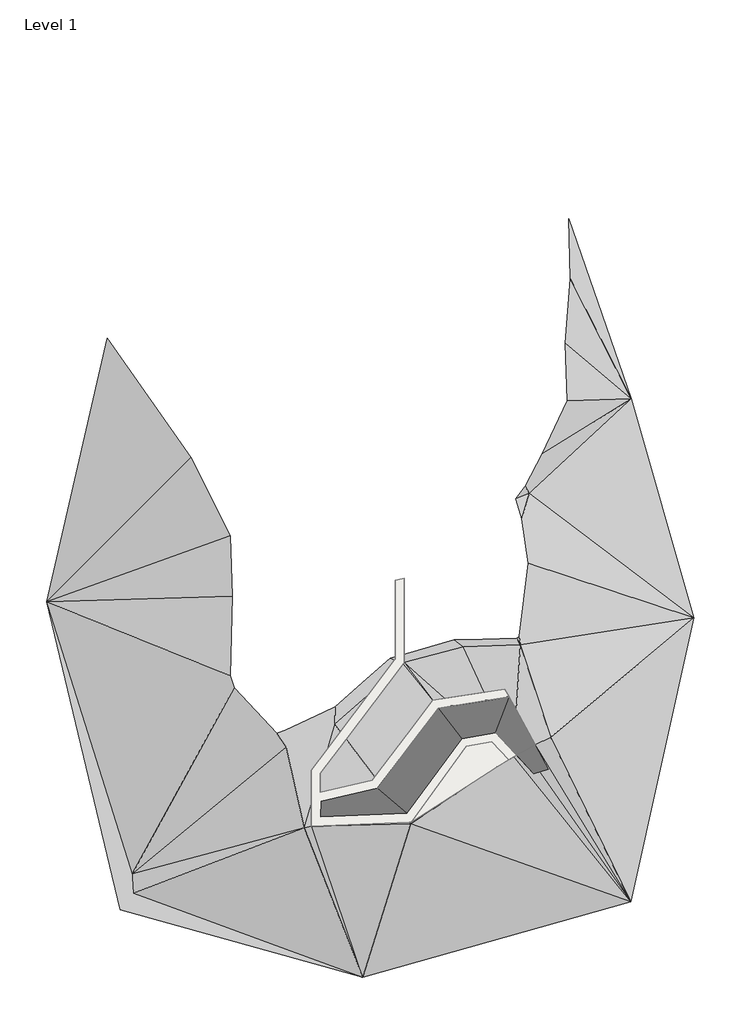
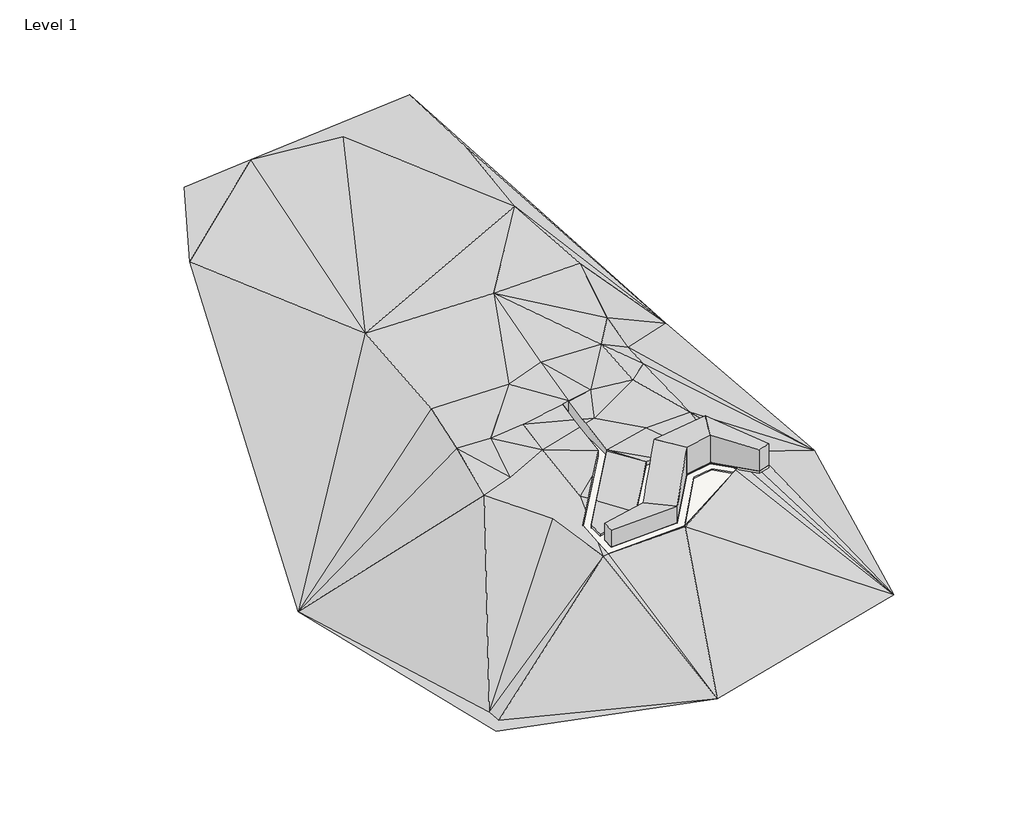
# One storey: 8 proxies, 4 slabs.
"""IFC4 building model written with IfcOpenShell, lengths in millimetres."""

import ifcopenshell
import ifcopenshell.guid

model = None  # the IFC model being written
_history = None  # IfcOwnerHistory: only IFC2X3 demands one
_inside = {}  # id of a spatial element -> (the spatial element, [elements in it])
_under = {}  # id of a project, library or spatial element -> (it, [spatial elements below it])
_declared = {}  # id of a project -> (the project, [libraries it declares])
_typed = {}  # id of a type object -> (the type object, [elements of that type])
_made_of = {}  # id of a material, layer set ... -> (it, [elements and type objects made of it])


def new_model(schema):
    """Start an empty IFC model of exactly this schema.

    Asked for "IFC4X3", IfcOpenShell would pick the latest addendum, in which some entities
    have other attributes; the version numbers below select the first issue.
    IFC2X3 requires an IfcOwnerHistory on every rooted entity: one is made here for all.
    """
    global model, _history
    if schema == "IFC4X3":
        model = ifcopenshell.file(schema_version=(4, 3, 0, 0))
    else:
        model = ifcopenshell.file(schema=schema)
    _inside.clear()
    _under.clear()
    _declared.clear()
    _typed.clear()
    _made_of.clear()
    _history = None
    if model.schema == "IFC2X3":
        org = make("IfcOrganization", Name="unknown")
        user = make(
            "IfcPersonAndOrganization",
            ThePerson=make("IfcPerson", FamilyName="unknown"),
            TheOrganization=org,
        )
        app = make(
            "IfcApplication",
            ApplicationDeveloper=org,
            Version="unknown",
            ApplicationFullName="unknown",
            ApplicationIdentifier="unknown",
        )
        _history = make(
            "IfcOwnerHistory",
            OwningUser=user,
            OwningApplication=app,
            ChangeAction="ADDED",
            CreationDate=0,
        )
    return model


def make(cls, **values):
    """One entity of the class cls with the attributes given. An attribute that is None is left unset."""
    return model.create_entity(
        cls, **{name: value for name, value in values.items() if value is not None}
    )


def rooted(cls, **values):
    """An entity with a GlobalId (a new one), such as an element, a storey or a relation."""
    return make(cls, GlobalId=ifcopenshell.guid.new(), OwnerHistory=_history, **values)


def si_unit(unit_type, name, prefix=None):
    """IfcSIUnit, for example si_unit("LENGTHUNIT", "METRE", prefix="MILLI")."""
    return make("IfcSIUnit", UnitType=unit_type, Prefix=prefix, Name=name)


def assignment(units):
    """IfcUnitAssignment: the units of a project."""
    return None if units is None else make("IfcUnitAssignment", Units=units)


def point(xyz):
    """IfcCartesianPoint."""
    return None if xyz is None else make("IfcCartesianPoint", Coordinates=xyz)


def direction(xyz):
    """IfcDirection."""
    return None if xyz is None else make("IfcDirection", DirectionRatios=xyz)


def frame(location, z_axis=None, x_axis=None):
    """IfcAxis2Placement3D, a coordinate frame: its origin and axes. An axis left out is left unset."""
    return make(
        "IfcAxis2Placement3D",
        Location=point(location),
        Axis=direction(z_axis),
        RefDirection=direction(x_axis),
    )


def origin():
    """The frame at (0, 0, 0) with its axes left unset."""
    return frame((0.0, 0.0, 0.0))


def place(relative_to, where):
    """IfcLocalPlacement: puts the frame where relative to a parent placement (None: the world)."""
    return make(
        "IfcLocalPlacement", PlacementRelTo=relative_to, RelativePlacement=where
    )


def context(
    kind, dimensions, precision=None, world=None, true_north=None, identifier=None
):
    """IfcGeometricRepresentationContext, for example the 3D "Model" context."""
    return make(
        "IfcGeometricRepresentationContext",
        ContextIdentifier=identifier,
        ContextType=kind,
        CoordinateSpaceDimension=dimensions,
        Precision=precision,
        WorldCoordinateSystem=world,
        TrueNorth=true_north,
    )


def project(units=None, contexts=None):
    """IfcProject with its units and contexts."""
    return rooted(
        "IfcProject",
        Name="project",
        RepresentationContexts=contexts,
        UnitsInContext=assignment(units),
    )


def spatial(cls, under=None, at=None, **own):
    """A site, building, storey or space (cls), placed at a placement, below another one or the project."""
    s = rooted(cls, ObjectPlacement=at, **own)
    if under is not None:
        _under.setdefault(under.id(), (under, []))[1].append(s)
    return s


def polyline(points):
    """IfcPolyline through the points."""
    return make("IfcPolyline", Points=[point(p) for p in points])


def point_list(points):
    """IfcCartesianPointList2D or 3D."""
    cls = (
        "IfcCartesianPointList2D" if len(points[0]) == 2 else "IfcCartesianPointList3D"
    )
    return make(cls, CoordList=points)


def outline(outer, holes=None, kind="AREA"):
    """IfcArbitraryClosedProfileDef: a profile drawn as a closed curve; with holes, ...WithVoids."""
    if holes is None:
        return make("IfcArbitraryClosedProfileDef", ProfileType=kind, OuterCurve=outer)
    return make(
        "IfcArbitraryProfileDefWithVoids",
        ProfileType=kind,
        OuterCurve=outer,
        InnerCurves=holes,
    )


def extrude(swept, where, along, depth):
    """IfcExtrudedAreaSolid: the profile swept, set in the frame where, extruded along a direction by depth."""
    return make(
        "IfcExtrudedAreaSolid",
        SweptArea=swept,
        Position=where,
        ExtrudedDirection=direction(along),
        Depth=depth,
    )


def triangles(points, corners, closed=None, point_numbers=None):
    """IfcTriangulatedFaceSet: each triangle names its three corners, points numbered from 1."""
    return make(
        "IfcTriangulatedFaceSet",
        Coordinates=point_list(points),
        Closed=closed,
        CoordIndex=corners,
        PnIndex=point_numbers,
    )


def shape(context_of_items, identifier, shape_type, items):
    """IfcShapeRepresentation: the items that make up one representation, for example the "Body"."""
    return make(
        "IfcShapeRepresentation",
        ContextOfItems=context_of_items,
        RepresentationIdentifier=identifier,
        RepresentationType=shape_type,
        Items=items,
    )


def made_of(thing, what):
    """Note that an element or type object is made of a material, layer set ...; save() writes the relation."""
    if what is not None:
        _made_of.setdefault(what.id(), (what, []))[1].append(thing)
    return thing


def element(
    cls,
    number,
    at=None,
    inside=None,
    cuts=None,
    type_object=None,
    material=None,
    context=None,
    identifier="Body",
    shape_type=None,
    held_by="IfcProductDefinitionShape",
    body=None,
    shapes=None,
    **own,
):
    """One element of the class cls, such as IfcWall. Its Tag is "e" and its number.

    at: its placement. inside: the storey or other place that contains it. cuts: it is an
    opening in that element (IfcRelVoidsElement). A single representation is given by context,
    identifier, shape_type and body (its items); several are given by shapes. held_by: the class
    of the entity that holds the representations. save() writes the other relations.
    """
    e = rooted(cls, Tag="e%d" % number, ObjectPlacement=at, **own)
    if body is not None:
        shapes = [shape(context, identifier, shape_type, body)]
    if shapes is not None:
        e.Representation = make(held_by, Representations=shapes)
    if inside is not None:
        _inside.setdefault(inside.id(), (inside, []))[1].append(e)
    if cuts is not None:
        rooted(
            "IfcRelVoidsElement", RelatingBuildingElement=cuts, RelatedOpeningElement=e
        )
    if type_object is not None:
        _typed.setdefault(type_object.id(), (type_object, []))[1].append(e)
    return made_of(e, material)


def aggregate(whole, parts):
    """IfcRelAggregates: a whole, such as a stair, and the parts it consists of."""
    return rooted("IfcRelAggregates", RelatingObject=whole, RelatedObjects=parts)


def save(model, path):
    """Write the relations noted so far, then the file.

    IfcRelAggregates (storeys below a building ...), IfcRelContainedInSpatialStructure (elements
    in a storey), IfcRelDefinesByType, IfcRelAssociatesMaterial and IfcRelDeclares: one each for
    every whole, place, type object, material and project.
    """
    for whole, parts in _under.values():
        aggregate(whole, parts)
    for where, things in _inside.values():
        rooted(
            "IfcRelContainedInSpatialStructure",
            RelatedElements=things,
            RelatingStructure=where,
        )
    for kind, things in _typed.values():
        rooted("IfcRelDefinesByType", RelatedObjects=things, RelatingType=kind)
    for what, things in _made_of.values():
        rooted("IfcRelAssociatesMaterial", RelatedObjects=things, RelatingMaterial=what)
    for by, libraries in _declared.values():
        rooted("IfcRelDeclares", RelatingContext=by, RelatedDefinitions=libraries)
    model.write(path)


def plane_surface(at):
    """IfcPlane: the flat surface through the origin of the frame at, square to its z axis."""
    return make("IfcPlane", Position=at)


def spline_surface(u_degree, v_degree, points, u_multiplicities, v_multiplicities, u_knots, v_knots, weights=None):
    """IfcBSplineSurfaceWithKnots; with weights, IfcRationalBSplineSurfaceWithKnots. points: one row for each step in u."""
    own = dict(
        UDegree=u_degree,
        VDegree=v_degree,
        ControlPointsList=[[point(p) for p in row] for row in points],
        SurfaceForm="UNSPECIFIED",
        UClosed=False,
        VClosed=False,
        SelfIntersect=False,
        UMultiplicities=u_multiplicities,
        VMultiplicities=v_multiplicities,
        UKnots=u_knots,
        VKnots=v_knots,
        KnotSpec="UNSPECIFIED",
    )
    if weights is None:
        return make("IfcBSplineSurfaceWithKnots", **own)
    return make("IfcRationalBSplineSurfaceWithKnots", WeightsData=weights, **own)


def advanced_brep(points, edges, surfaces, faces):
    """IfcAdvancedBrep: a solid bounded by faces that lie on surfaces and meet in shared edges.

    An edge is (start, end): straight between two places in points (the first is 0);
    or (start, end, curve); or (start, end, curve, False) where it runs against its curve.
    A face is (place in surfaces, loops), or (place, loops, False) where it looks against
    its surface's normal. A loop lists edges by number (the first is 1), with a minus sign
    where the edge is run from its end to its start. The first loop is the outer one.
    """
    corners = [point(p) for p in points]
    vertices = [make("IfcVertexPoint", VertexGeometry=c) for c in corners]
    made = []
    for start, end, *more in edges:
        made.append(
            make(
                "IfcEdgeCurve",
                EdgeStart=vertices[start],
                EdgeEnd=vertices[end],
                EdgeGeometry=more[0] if more else make("IfcPolyline", Points=[corners[start], corners[end]]),
                SameSense=more[1] if len(more) > 1 else True,
            )
        )
    hull = []
    for where, loops, *sense in faces:
        bounds = []
        for j, loop in enumerate(loops):
            ring = [make("IfcOrientedEdge", EdgeElement=made[abs(k) - 1], Orientation=k > 0) for k in loop]
            bounds.append(
                make(
                    "IfcFaceOuterBound" if j == 0 else "IfcFaceBound",
                    Bound=make("IfcEdgeLoop", EdgeList=ring),
                    Orientation=True,
                )
            )
        hull.append(make("IfcAdvancedFace", Bounds=bounds, FaceSurface=surfaces[where], SameSense=sense[0] if sense else True))
    return make("IfcAdvancedBrep", Outer=make("IfcClosedShell", CfsFaces=hull))


model = new_model("IFC4")

# Units and contexts
model_context = context("Model", 3, world=origin())
ifc_project = project(units=[si_unit("LENGTHUNIT", "METRE", prefix="MILLI")], contexts=[model_context])

# Site, building, storey
site = spatial("IfcSite", under=ifc_project)
building = spatial("IfcBuilding", under=site)
storey = spatial("IfcBuildingStorey", under=building, Name="Level 1", Elevation=16000.0)

# Proxies
placement = place(None, origin())
element("IfcBuildingElementProxy", 1, Name="Building Element Proxy", at=placement, inside=storey, context=model_context, shape_type="Tessellation", body=[
    triangles([(25163.1129089, -22515.1373291, 0.0), (33501.38302, 14958.2323151, 0.0), (25213.2424072, 43856.3509644, 8000.000061), (9088.2592163, 90310.3945312, 25999.9990356), (-19208.4752106, 87582.0587402, 25999.9990356), (-30997.5800354, 86417.4135498, 25999.9990356), (-39784.0692993, 69640.2887695, 25999.9990356), (-51893.8324585, 17101.8572845, 0.0), (-42165.2867432, -23534.0821106, 0.0), (-10201.0947784, -32468.2530579, 0.0), (-3787.8249001, -11972.8750031, 16008.6123871), (-3883.804216, -11976.7910431, 16011.3366394), (-4050.2638229, -11983.5848145, 16017.6734619), (-16964.3563751, -12510.5945068, 16012.8679413), (-16964.3563751, -9508.5626312, 16235.2485535), (-16964.3563751, -5151.2425507, 16605.8596527), (-14866.6053497, -2370.5932377, 16758.4456879), (-13135.0145325, -75.3026574, 16923.8821014), (-9432.1132278, 4833.0349388, 16999.9995483), (-6004.6020905, 9376.3329117, 17135.7633545), (-5919.4090347, 9489.2591583, 17149.4939117), (-5919.4090347, 14896.12099, 18000.0001373), (-5919.4090347, 16517.4406311, 18283.0084442), (-5919.4090347, 19908.1871521, 18999.0414825), (-5816.0903412, 19933.9460449, 18999.9995636), (-4719.4093163, 20207.3805176, 19005.925946), (-4719.4093163, 20159.1881104, 18999.9995636), (-4719.4093163, 16217.0926849, 18167.5375854), (-4719.4093163, 15257.2942932, 18000.0001373), (-4719.4093163, 9242.8329208, 17053.9171875), (-4719.4093163, 9087.3802002, 17029.5640228), (-4783.3841904, 9002.578981, 17019.1541931), (-4867.5130669, 8891.0631134, 17005.5957184), (-5008.7774094, 8703.8117523, 16999.9995483), (-12379.2211304, -1065.9950346, 16848.4913544), (-15764.356366, -5553.1209274, 16525.0738861), (-15764.356366, -8050.3853577, 16340.0851776), (-8936.3510468, -6464.9617813, 16439.427951), (-8600.257608, -6019.4569977, 16471.537619), (-4400.5758705, -452.6177579, 16557.8672333), (-977.7347242, 4084.4896408, 16663.3084717), (596.0196516, 4328.2267982, 16626.9153442), (5823.6369736, 5137.860228, 16584.7039673), (8545.2801498, 5559.3781036, 16607.2456146), (9145.2801544, 4520.1473511, 16534.9825836), (6308.3591309, 4080.775914, 16511.4863434), (1735.345966, 3372.5249588, 16548.4131592), (-242.7929745, 3066.1584846, 16594.1568787), (-4316.2391579, -2333.3511795, 16468.6738403), (-7844.4647873, -7010.1494339, 16396.1468719), (-8238.3535355, -7532.2640762, 16358.515448), (-8229.1552597, -7530.1281601, 16358.6491608), (-7840.6499039, -7015.1497101, 16395.7666626), (-4315.8136024, -2342.8437687, 16468.2238678), (-244.6116317, 3053.6909317, 16593.6383057), (1747.6090256, 3362.2383774, 16547.5678619), (6313.5762543, 4069.3981201, 16510.6991821), (9152.0739258, 4509.0137283, 16534.2082123), (10063.5148041, 2818.8947983, 16416.8339813), (12554.0558075, -1799.4121136, 16002.4534607), (11175.695755, -2542.7282249, 16000.0001221), (10089.6108856, -3128.4276489, 15983.7906464), (10072.26427, -3109.8264587, 16000.0001221), (9728.4957184, -2741.1797745, 16038.3117371), (9154.0860123, -2125.200222, 16081.6428131), (7327.6009872, -166.5349657, 16233.6033051), (7322.7018677, -167.4168159, 16233.6346985), (9159.6205582, -2137.2711422, 16080.8068176), (9728.1486465, -2746.9427948, 16037.9187378), (10068.3970642, -3111.8141281, 16000.0001221), (10099.6567841, -3145.3365005, 15970.7891144), (9735.9627045, -3355.3158348, 15957.2038971), (9052.6648773, -3749.8179176, 15986.7939514), (7578.7676331, -4693.7024551, 16000.0001221), (-40587.1272583, -18814.4155426, 0.0), (-25319.0708313, 43678.385083, 24000.0001831), (10546.016748, 43439.8275513, 24000.0001831), (14580.0833038, -793.0747021, 16000.0001221), (-24826.3613708, 17881.2527344, 18999.9995636), (-19286.2972046, 17611.0355072, 18999.9995636), (9352.4954132, 22907.8714966, 18999.9995636), (9544.3464935, 74843.7153442, 25999.9990356), (8215.5142319, 58226.1529175, 25999.9990356), (-4109.1041267, 43103.3318115, 24000.0001831), (-4648.2401138, 85919.8997314, 25999.9990356), (10579.6565552, 11384.9539124, 16999.9995483), (-26544.1123352, 6881.1846313, 18000.0001373), (-562.7335656, 21012.9080933, 18999.9995636), (-17907.5836853, -12718.0620758, 16000.0001221), (-13370.5106232, 18382.3814484, 18999.9995636), (-20280.9178894, -2077.2245167, 16999.9995483), (-13898.0935364, 924.940781, 16999.9995483), (-4818.6334923, 8870.2027588, 16999.9995483), (3074.2245621, 11133.7936615, 16999.9995483), (6032.5701508, 20211.7895508, 18999.9995636), (-2978.3339035, 15781.3181213, 18000.0001373), (-13554.1819702, 12598.2298553, 18000.0001373), (-21011.2942383, 8906.3772949, 18000.0001373), (-23725.2820679, 27223.545282, 20000.0001526), (-10876.5675018, 27027.3107483, 20000.0001526), (-4019.0860748, 29531.4695251, 20000.0001526), (9952.9645752, 34368.7905396, 20000.0001526), (5864.755394, 29059.2239319, 20000.0001526), (11773.534845, 31391.5234314, 16000.0001221), (-40428.1090576, -21350.1851807, 0.0), (-3873.0853935, -12215.8299408, 16000.0001221)], [[9, 105, 75], [89, 105, 10], [75, 105, 89], [9, 75, 8], [89, 14, 15], [10, 14, 89], [75, 89, 91], [10, 105, 9], [91, 89, 15], [91, 98, 87], [91, 87, 75], [91, 15, 16], [17, 91, 16], [36, 38, 35], [17, 92, 91], [18, 92, 17], [38, 36, 37], [92, 98, 91], [75, 87, 8], [52, 53, 50], [49, 50, 54], [52, 50, 51], [50, 53, 54], [35, 40, 34], [18, 19, 92], [41, 93, 34], [93, 41, 31], [40, 35, 39], [35, 38, 39], [97, 92, 19], [14, 10, 106], [33, 34, 93], [87, 79, 8], [79, 87, 98], [79, 98, 80], [8, 79, 99], [90, 80, 97], [97, 80, 98], [97, 98, 92], [22, 90, 97], [20, 97, 19], [79, 80, 99], [6, 7, 5], [7, 8, 76], [5, 7, 76], [100, 99, 80], [24, 100, 90], [100, 76, 99], [5, 76, 85], [83, 85, 76], [100, 80, 90], [8, 99, 76], [20, 21, 97], [23, 90, 22], [31, 32, 93], [29, 30, 96], [31, 94, 30], [33, 93, 32], [24, 90, 23], [26, 100, 25], [27, 28, 96], [100, 84, 76], [88, 26, 27], [28, 29, 96], [25, 100, 24], [26, 101, 100], [22, 97, 21], [5, 85, 4], [41, 34, 40], [13, 106, 12], [106, 13, 14], [12, 106, 11], [106, 74, 11], [73, 74, 1], [74, 106, 1], [49, 54, 55], [67, 65, 66], [55, 47, 48], [68, 65, 67], [70, 62, 63], [70, 63, 69], [61, 62, 71], [71, 62, 70], [1, 71, 72], [61, 71, 1], [72, 73, 1], [68, 69, 64], [69, 63, 64], [61, 1, 60], [59, 78, 86], [78, 59, 60], [1, 78, 60], [68, 64, 65], [1, 2, 78], [106, 10, 1], [42, 94, 31], [46, 56, 57], [44, 94, 43], [46, 47, 56], [55, 56, 47], [42, 43, 94], [103, 84, 101], [84, 100, 101], [27, 96, 88], [101, 26, 88], [95, 88, 96], [86, 95, 94], [88, 103, 101], [103, 88, 95], [95, 81, 103], [95, 96, 94], [30, 94, 96], [84, 103, 102], [41, 42, 31], [45, 57, 58], [44, 45, 86], [44, 86, 94], [81, 95, 86], [58, 59, 86], [81, 2, 104], [2, 81, 86], [78, 2, 86], [86, 45, 58], [103, 81, 104], [4, 85, 82], [82, 83, 3], [4, 82, 3], [83, 82, 85], [102, 104, 3], [102, 103, 104], [77, 3, 83], [3, 77, 102], [104, 2, 3], [77, 83, 84], [102, 77, 84], [46, 57, 45], [76, 84, 83], [48, 49, 55]], closed=False),
])
element("IfcBuildingElementProxy", 2, Name="Building Element Proxy", at=placement, inside=storey, context=model_context, shape_type="Tessellation", body=[
    triangles([(7322.7018677, -167.4168159, 15695.0408295), (7322.7018677, -167.4168159, 16233.6346985), (7327.6009872, -166.5349657, 15695.0408295), (7327.6009872, -166.5349657, 16233.6033051), (9154.0860123, -2125.200222, 15695.0408295), (9154.0860123, -2125.200222, 16081.6428131), (9728.4957184, -2741.1797745, 15695.0408295), (9728.4957184, -2741.1797745, 16038.3117371), (10072.26427, -3109.8264587, 15695.0408295), (10072.26427, -3109.8264587, 16000.0001221), (10089.6108856, -3128.4276489, 15695.0408295), (10089.6108856, -3128.4276489, 15983.7906464), (11175.695755, -2542.7282249, 15695.0408295), (11175.695755, -2542.7282249, 16000.0001221), (12554.0558075, -1799.4121136, 15695.0408295), (12554.0558075, -1799.4121136, 16002.4534607), (10063.5148041, 2818.8947983, 15695.0408295), (10063.5148041, 2818.8947983, 16416.8339813), (9152.0739258, 4509.0137283, 15695.0408295), (9152.0739258, 4509.0137283, 16534.2082123), (6313.5762543, 4069.3981201, 15695.0408295), (6313.5762543, 4069.3981201, 16510.6991821), (1747.6090256, 3362.2383774, 15695.0408295), (1747.6090256, 3362.2383774, 16547.5678619), (-244.6116317, 3053.6909317, 15695.0408295), (-244.6116317, 3053.6909317, 16593.6383057), (-4315.8136024, -2342.8437687, 15695.0408295), (-4315.8136024, -2342.8437687, 16468.2238678), (-7840.6499039, -7015.1497101, 15695.0408295), (-7840.6499039, -7015.1497101, 16395.7666626), (-8229.1552597, -7530.1281601, 15695.0408295), (-8229.1552597, -7530.1281601, 16358.6491608), (-8238.3535355, -7532.2640762, 15695.0408295), (-8238.3535355, -7532.2640762, 16358.515448)], [[1, 4, 2], [1, 3, 4], [3, 6, 4], [3, 5, 6], [5, 8, 6], [5, 7, 8], [7, 10, 8], [7, 9, 10], [9, 12, 10], [9, 11, 12], [11, 14, 12], [11, 13, 14], [13, 16, 14], [13, 15, 16], [15, 18, 16], [15, 17, 18], [17, 20, 18], [17, 19, 20], [19, 22, 20], [19, 21, 22], [21, 24, 22], [21, 23, 24], [23, 26, 24], [23, 25, 26], [25, 28, 26], [25, 27, 28], [27, 30, 28], [27, 29, 30], [29, 32, 30], [29, 31, 32], [31, 34, 32], [31, 33, 34]], closed=False),
    triangles([(-15687.0227142, -9261.8026932, 15695.0408295), (-15756.8207794, -11260.5847595, 15695.0408295), (-4355.2341614, -10785.3463257, 15695.0408295), (2854.3455414, -971.75522, 15695.0408295), (7327.6009872, -166.5349657, 15695.0408295), (10089.6108856, -3128.4276489, 15695.0408295), (12554.0558075, -1799.4121136, 15695.0408295), (9152.0739258, 4509.0137283, 15695.0408295), (-244.6116317, 3053.6909317, 15695.0408295), (-8229.1552597, -7530.1281601, 15695.0408295)], [[2, 3, 10], [10, 1, 2], [4, 9, 10], [10, 3, 4], [6, 7, 5], [5, 8, 9], [8, 5, 7], [5, 9, 4]], closed=False),
])
element("IfcBuildingElementProxy", 3, Name="Building Element Proxy", at=placement, inside=storey, context=model_context, shape_type="Tessellation", body=[
    triangles([(9052.6648773, -3749.8179176, 15695.0408295), (9052.6648773, -3749.8179176, 15986.7939514), (9735.9627045, -3355.3158348, 15695.0408295), (9735.9627045, -3355.3158348, 15957.2038971), (10099.6567841, -3145.3365005, 15695.0408295), (10099.6567841, -3145.3365005, 15970.7891144), (10068.3970642, -3111.8141281, 15695.0408295), (10068.3970642, -3111.8141281, 16000.0001221), (9728.1486465, -2746.9427948, 15695.0408295), (9728.1486465, -2746.9427948, 16037.9187378), (9159.6205582, -2137.2711422, 15695.0408295), (9159.6205582, -2137.2711422, 16080.8068176), (7322.7018677, -167.4168159, 15695.0408295), (7322.7018677, -167.4168159, 16233.6346985)], [[1, 4, 2], [1, 3, 4], [3, 6, 4], [3, 5, 6], [5, 8, 6], [5, 7, 8], [7, 10, 8], [7, 9, 10], [9, 12, 10], [9, 11, 12], [11, 14, 12], [11, 13, 14]], closed=False),
    triangles([(-3787.8249001, -11972.8750031, 15695.0408295), (-3787.8249001, -11972.8750031, 16008.6123871), (-3883.804216, -11976.7910431, 15695.0408295), (-3883.804216, -11976.7910431, 16011.3366394), (-4050.2638229, -11983.5848145, 15695.0408295), (-4050.2638229, -11983.5848145, 16017.6734619), (-16964.3563751, -12510.5945068, 15695.0408295), (-16964.3563751, -12510.5945068, 16012.8679413), (-16964.3563751, -9508.5626312, 15695.0408295), (-16964.3563751, -9508.5626312, 16235.2485535), (-16964.3563751, -5151.2425507, 15695.0408295), (-16964.3563751, -5151.2425507, 16605.8596527), (-14866.6053497, -2370.5932377, 15695.0408295), (-14866.6053497, -2370.5932377, 16758.4456879), (-13135.0145325, -75.3026574, 15695.0408295), (-13135.0145325, -75.3026574, 16923.8821014), (-9432.1132278, 4833.0349388, 15695.0408295), (-9432.1132278, 4833.0349388, 16999.9995483), (-6004.6020905, 9376.3329117, 15695.0408295), (-6004.6020905, 9376.3329117, 17135.7633545), (-5919.4090347, 9489.2591583, 15695.0408295), (-5919.4090347, 9489.2591583, 17149.4939117), (-5919.4090347, 14896.12099, 15695.0408295), (-5919.4090347, 14896.12099, 18000.0001373), (-5919.4090347, 16517.4406311, 15695.0408295), (-5919.4090347, 16517.4406311, 18283.0084442), (-5919.4090347, 19908.1871521, 15695.0408295), (-5919.4090347, 19908.1871521, 18999.0414825), (-5816.0903412, 19933.9460449, 15695.0408295), (-5816.0903412, 19933.9460449, 18999.9995636), (-4719.4093163, 20207.3805176, 15695.0408295), (-4719.4093163, 20207.3805176, 19005.925946), (-4719.4093163, 20159.1881104, 15695.0408295), (-4719.4093163, 20159.1881104, 18999.9995636), (-4719.4093163, 16217.0926849, 15695.0408295), (-4719.4093163, 16217.0926849, 18167.5375854), (-4719.4093163, 15257.2942932, 15695.0408295), (-4719.4093163, 15257.2942932, 18000.0001373), (-4719.4093163, 9242.8329208, 15695.0408295), (-4719.4093163, 9242.8329208, 17053.9171875), (-4719.4093163, 9087.3802002, 15695.0408295), (-4719.4093163, 9087.3802002, 17029.5640228), (-4783.3841904, 9002.578981, 15695.0408295), (-4783.3841904, 9002.578981, 17019.1541931), (-4867.5130669, 8891.0631134, 15695.0408295), (-4867.5130669, 8891.0631134, 17005.5957184), (-5008.7774094, 8703.8117523, 15695.0408295), (-5008.7774094, 8703.8117523, 16999.9995483), (-12379.2211304, -1065.9950346, 15695.0408295), (-12379.2211304, -1065.9950346, 16848.4913544), (-15764.356366, -5553.1209274, 15695.0408295), (-15764.356366, -5553.1209274, 16525.0738861), (-15764.356366, -8050.3853577, 15695.0408295), (-15764.356366, -8050.3853577, 16340.0851776), (-8936.3510468, -6464.9617813, 15695.0408295), (-8936.3510468, -6464.9617813, 16439.427951), (-8600.257608, -6019.4569977, 15695.0408295), (-8600.257608, -6019.4569977, 16471.537619), (-4400.5758705, -452.6177579, 15695.0408295), (-4400.5758705, -452.6177579, 16557.8672333), (-977.7347242, 4084.4896408, 15695.0408295), (-977.7347242, 4084.4896408, 16663.3084717), (596.0196516, 4328.2267982, 15695.0408295), (596.0196516, 4328.2267982, 16626.9153442), (5823.6369736, 5137.860228, 15695.0408295), (5823.6369736, 5137.860228, 16584.7039673), (8545.2801498, 5559.3781036, 15695.0408295), (8545.2801498, 5559.3781036, 16607.2456146), (9145.2801544, 4520.1473511, 15695.0408295), (9145.2801544, 4520.1473511, 16534.9825836), (6308.3591309, 4080.775914, 15695.0408295), (6308.3591309, 4080.775914, 16511.4863434), (1735.345966, 3372.5249588, 15695.0408295), (1735.345966, 3372.5249588, 16548.4131592), (-242.7929745, 3066.1584846, 15695.0408295), (-242.7929745, 3066.1584846, 16594.1568787), (-4316.2391579, -2333.3511795, 15695.0408295), (-4316.2391579, -2333.3511795, 16468.6738403), (-7844.4647873, -7010.1494339, 15695.0408295), (-7844.4647873, -7010.1494339, 16396.1468719), (-8238.3535355, -7532.2640762, 15695.0408295), (-8238.3535355, -7532.2640762, 16358.515448)], [[1, 4, 2], [1, 3, 4], [3, 6, 4], [3, 5, 6], [5, 8, 6], [5, 7, 8], [7, 10, 8], [7, 9, 10], [9, 12, 10], [9, 11, 12], [11, 14, 12], [11, 13, 14], [13, 16, 14], [13, 15, 16], [15, 18, 16], [15, 17, 18], [17, 20, 18], [17, 19, 20], [19, 22, 20], [19, 21, 22], [21, 24, 22], [21, 23, 24], [23, 26, 24], [23, 25, 26], [25, 28, 26], [25, 27, 28], [27, 30, 28], [27, 29, 30], [29, 32, 30], [29, 31, 32], [31, 34, 32], [31, 33, 34], [33, 36, 34], [33, 35, 36], [35, 38, 36], [35, 37, 38], [37, 40, 38], [37, 39, 40], [39, 42, 40], [39, 41, 42], [41, 44, 42], [41, 43, 44], [43, 46, 44], [43, 45, 46], [45, 48, 46], [45, 47, 48], [47, 50, 48], [47, 49, 50], [49, 52, 50], [49, 51, 52], [51, 54, 52], [51, 53, 54], [53, 56, 54], [53, 55, 56], [55, 58, 56], [55, 57, 58], [57, 60, 58], [57, 59, 60], [59, 62, 60], [59, 61, 62], [61, 64, 62], [61, 63, 64], [63, 66, 64], [63, 65, 66], [65, 68, 66], [65, 67, 68], [67, 70, 68], [67, 69, 70], [69, 72, 70], [69, 71, 72], [71, 74, 72], [71, 73, 74], [73, 76, 74], [73, 75, 76], [75, 78, 76], [75, 77, 78], [77, 80, 78], [77, 79, 80], [79, 82, 80], [79, 81, 82]], closed=False),
    triangles([(-16964.3563751, -12510.5945068, 15695.0408295), (-3787.8249001, -11972.8750031, 15695.0408295), (3484.4704514, -1969.9799, 15695.0408295), (6841.0283615, -1378.1282352, 15695.0408295), (9052.6648773, -3749.8179176, 15695.0408295), (10099.6567841, -3145.3365005, 15695.0408295), (7322.7018677, -167.4168159, 15695.0408295), (2859.9347351, -970.7491041, 15695.0408295), (-4351.2928322, -10786.5834595, 15695.0408295), (-15752.4919739, -11261.8056152, 15695.0408295), (-15682.7043732, -9263.3502731, 15695.0408295), (-8240.6859512, -7535.355748, 15695.0408295), (-242.7929745, 3066.1584846, 15695.0408295), (9145.2801544, 4520.1473511, 15695.0408295), (8545.2801498, 5559.3781036, 15695.0408295), (-977.7347242, 4084.4896408, 15695.0408295), (-8936.3510468, -6464.9617813, 15695.0408295), (-15764.356366, -8050.3853577, 15695.0408295), (-15764.356366, -5553.1209274, 15695.0408295), (-4719.4093163, 9087.3802002, 15695.0408295), (-4719.4093163, 20207.3805176, 15695.0408295), (-5919.4090347, 19908.1871521, 15695.0408295), (-5919.4090347, 9489.2591583, 15695.0408295), (-16964.3563751, -5151.2425507, 15695.0408295)], [[18, 1, 11], [11, 1, 10], [1, 18, 24], [11, 12, 17], [11, 17, 18], [10, 1, 2], [19, 24, 18], [23, 24, 19], [23, 20, 21], [23, 21, 22], [19, 20, 23], [9, 2, 3], [2, 9, 10], [9, 3, 8], [4, 5, 6], [4, 6, 7], [3, 4, 8], [15, 16, 13], [16, 17, 13], [17, 12, 13], [14, 15, 13], [8, 4, 7]], closed=False),
])
element("IfcBuildingElementProxy", 4, Name="Building Element Proxy", at=placement, inside=storey, context=model_context, shape_type="Tessellation", body=[
    triangles([(9052.6648773, -3749.8179176, 15495.0402466), (9052.6648773, -3749.8179176, 15695.0408295), (9038.6459656, -3734.7842422, 15495.0402466), (9038.6459656, -3734.7842422, 15695.0408295), (6841.0283615, -1378.1282352, 15495.0402466), (6841.0283615, -1378.1282352, 15695.0408295), (3484.4704514, -1969.9799, 15495.0402466), (3484.4704514, -1969.9799, 15695.0408295), (-3787.8249001, -11972.8750031, 15495.0402466), (-3787.8249001, -11972.8750031, 15695.0408295)], [[1, 4, 2], [1, 3, 4], [3, 6, 4], [3, 5, 6], [5, 8, 6], [5, 7, 8], [7, 10, 8], [7, 9, 10]], closed=False),
    triangles([(9052.6648773, -3749.8179176, 15495.0402466), (9052.6648773, -3749.8179176, 15986.7939514), (7578.7676331, -4693.7024551, 15495.0402466), (7578.7676331, -4693.7024551, 16000.0001221), (-3787.8249001, -11972.8750031, 15495.0402466), (-3787.8249001, -11972.8750031, 16008.6123871)], [[1, 4, 2], [1, 3, 4], [3, 6, 4], [3, 5, 6]], closed=False),
    triangles([(9052.6648773, -3749.8179176, 15495.0402466), (6841.0283615, -1378.1282352, 15495.0402466), (3484.4704514, -1969.9799, 15495.0402466), (-3787.8249001, -11972.8750031, 15495.0402466)], [[3, 4, 1], [1, 2, 3]], closed=False),
])
element("IfcBuildingElementProxy", 5, Name="Mass 1 : Mass 1", ObjectType="Mass 1 : Mass 1", at=placement, inside=storey, context=model_context, shape_type="AdvancedBrep", body=[
    advanced_brep(
    [(12369.2980289, -5573.0932179, 16000.0), (14291.8214208, -5021.8185063, 16000.0), (14291.8214208, -5021.8185063, 20000.0), (12369.2980289, -5573.0932179, 20000.0), (9148.9033844, 4514.8933577, 16000.0), (9148.9033844, 4514.8933577, 21000.0), (7322.5101644, -161.0758259, 16000.0), (7322.5101644, -161.0758259, 21000.0)],
    [
        (0, 1),
        (1, 2),
        (2, 3),
        (3, 0),
        (1, 4),
        (4, 5),
        (5, 2),
        (4, 6),
        (6, 7),
        (7, 5),
        (6, 0),
        (3, 7),
    ],
    [
        plane_surface(frame((13330.5597248, -5297.4558621, 16000.0), z_axis=(0.2756373558169583, -0.9612616959383306, 0.0), x_axis=(0.9612616959383306, 0.2756373558169583, 0.0))),
        plane_surface(frame((11720.3624026, -253.4625743, 16000.0), z_axis=(0.8801717513645727, 0.47465533611223737, 0.0), x_axis=(-0.4726466032472634, 0.8764468803070403, 0.09190241802521144))),
        plane_surface(frame((8235.7067744, 2176.9087659, 16000.0), z_axis=(-0.9314679648616316, 0.36382335059274323, 0.0), x_axis=(-0.36382335059274323, -0.9314679648616316, 0.0))),
        plane_surface(frame((9845.9040967, -2867.0845219, 16000.0), z_axis=(-0.7313537016191938, -0.6819983600624737, 0.0), x_axis=(0.6758552123741655, -0.7247659822571911, -0.13391789600139645))),
        spline_surface(1, 1, [[(9148.9033844, 4514.8933577, 21000.0), (14291.8214208, -5021.8185063, 20000.0)], [(7322.5101644, -161.0758259, 21000.0), (12369.2980289, -5573.0932179, 20000.0)]], [2, 2], [2, 2], [0.0, 1.0], [0.0, 1.0]),
        plane_surface(frame((10783.1332496, -1560.2735481, 16000.0), z_axis=(0.0, 0.0, -1.0), x_axis=(-0.6819983600624736, 0.7313537016191938, 0.0))),
    ],
    [
        (0, [[1, 2, 3, 4]]),
        (1, [[5, 6, 7, -2]]),
        (2, [[8, 9, 10, -6]]),
        (3, [[11, -4, 12, -9]]),
        (4, [[-7, -10, -12, -3]]),
        (5, [[-11, -8, -5, -1]]),
    ],
),
])
element("IfcBuildingElementProxy", 6, Name="Mass 11 : Mass 2", ObjectType="Mass 11 : Mass 2", at=placement, inside=storey, context=model_context, shape_type="SweptSolid", body=[
    extrude(outline(polyline([(-238.9778756, 3054.5633259), (9149.0951885, 4508.5523712), (7322.7019685, -167.4168124), (2859.9348278, -970.7490914), (-238.9778756, 3054.5633259)])), frame((0.0, 0.0, 16000.0), z_axis=(0.0, 0.0, 1.0), x_axis=(1.0, 0.0, 0.0)), (0.0, 0.0, 1.0), 5000.0),
])
element("IfcBuildingElementProxy", 7, Name="Mass 12 : Mass 4", ObjectType="Mass 12 : Mass 4", at=placement, inside=storey, context=model_context, shape_type="SweptSolid", body=[
    extrude(outline(polyline([(-15756.8212688, -11260.5843485), (-15687.0222753, -9261.8026945), (-8242.8962803, -7533.3189626), (-4366.7113981, -10785.8242677), (-15756.8212688, -11260.5843485)])), frame((0.0, 0.0, 16000.0), z_axis=(0.0, 0.0, 1.0), x_axis=(1.0, 0.0, 0.0)), (0.0, 0.0, 1.0), 3000.0),
])
element("IfcBuildingElementProxy", 8, Name="Mass 3 : Mass 3", ObjectType="Mass 3 : Mass 3", at=placement, inside=storey, context=model_context, shape_type="AdvancedBrep", body=[
    advanced_brep(
    [(-4363.3257058, -10796.3600032, 16000.0), (2859.7430237, -964.408105, 16000.0), (2859.7430237, -964.408105, 21000.0), (-4363.3257058, -10796.3600032, 19000.0), (-239.1696796, 3060.9043124, 16000.0), (-239.1696796, 3060.9043124, 21000.0), (-8239.510588, -7543.8546982, 16000.0), (-8239.510588, -7543.8546982, 19000.0)],
    [
        (0, 1),
        (1, 2),
        (2, 3),
        (3, 0),
        (1, 4),
        (4, 5),
        (5, 2),
        (4, 6),
        (6, 7),
        (7, 5),
        (6, 0),
        (3, 7),
    ],
    [
        plane_surface(frame((-751.791341, -5880.3840541, 16000.0), z_axis=(0.8058976965757628, -0.5920548138930045, 0.0), x_axis=(0.5842560696085248, 0.7952821422257879, 0.16177502706648056))),
        plane_surface(frame((1310.286672, 1048.2481037, 16000.0), z_axis=(0.79238433411756, 0.6100221856990702, 0.0), x_axis=(-0.6100221856990702, 0.79238433411756, 0.0))),
        plane_surface(frame((-4239.3401338, -2241.4751929, 16000.0), z_axis=(-0.7983068021215491, 0.6022509856251511, 0.0), x_axis=(-0.5955392011731624, -0.7894100741621346, -0.14887845605514874))),
        plane_surface(frame((-6301.4181469, -9170.1073507, 16000.0), z_axis=(-0.642787609686557, -0.7660444431189631, 0.0), x_axis=(0.7660444431189631, -0.642787609686557, 0.0))),
        spline_surface(1, 1, [[(-4363.3257058, -10796.3600032, 19000.0), (-8239.510588, -7543.8546982, 19000.0)], [(2859.7430237, -964.408105, 21000.0), (-239.1696796, 3060.9043124, 21000.0)]], [2, 2], [2, 2], [0.0, 1.0], [0.0, 1.0]),
        plane_surface(frame((-2495.5657374, -4060.9296235, 16000.0), z_axis=(0.0, 0.0, -1.0), x_axis=(-0.7660444431189647, 0.6427876096865552, 0.0))),
    ],
    [
        (0, [[1, 2, 3, 4]]),
        (1, [[5, 6, 7, -2]]),
        (2, [[8, 9, 10, -6]]),
        (3, [[11, -4, 12, -9]]),
        (4, [[-12, -3, -7, -10]]),
        (5, [[-11, -8, -5, -1]]),
    ],
),
])

# Slabs
element("IfcSlab", 9, ObjectType="Generic Floor - 400mm", at=placement, inside=storey, context=model_context, shape_type="SweptSolid", body=[
    extrude(outline(polyline([(-8242.8962803, -7533.3189626), (-257.4450567, 3051.7031991), (9151.9538082, 4508.9951033), (14291.7085175, -5021.8508808), (12364.783837, -5574.3876416), (7322.7019685, -167.4168124), (2843.629872, -973.6841084), (-4355.5531236, -10773.1230408), (-15745.6629942, -11247.8831217), (-15676.2199478, -9259.2944555), (-8242.8962803, -7533.3189626)])), frame((0.0, 0.0, 15800.0), z_axis=(0.0, 0.0, 1.0), x_axis=(1.0, 0.0, 0.0)), (0.0, 0.0, 1.0), 400.0),
])
element("IfcSlab", 10, ObjectType="Pad 1", at=placement, inside=storey, context=model_context, shape_type="SweptSolid", body=[
    extrude(outline(polyline([(-15687.0222753, -9261.8026945), (-8229.1553171, -7530.1283891), (-244.6116358, 3053.6907905), (9152.0741216, 4509.013737), (12554.0556042, -1799.4121287), (10089.6105749, -3128.4277236), (7327.6008966, -166.5349678), (2854.3454443, -971.7552233), (-4355.2341485, -10785.3458754), (-15756.8212688, -11260.5843485), (-15687.0222753, -9261.8026945)])), frame((0.0, 0.0, 15695.2), z_axis=(0.0, 0.0, 1.0), x_axis=(1.0, 0.0, 0.0)), (0.0, 0.0, 1.0), 304.8),
])
element("IfcSlab", 11, ObjectType="Pad 1", at=placement, inside=storey, context=model_context, shape_type="SweptSolid", body=[
    extrude(outline(polyline([(-16964.3562895, -12510.593954), (-16964.3562895, -5151.2424708), (-5919.409228, 9489.2588795), (-5919.409228, 19908.1865856), (-4719.409228, 20207.380189), (-4719.409228, 9087.380189), (-15764.3562895, -5553.1211613), (-15764.3562895, -8050.3855576), (-8936.3507581, -6464.9614944), (-977.7347491, 4084.4895602), (8545.2800949, 5559.3778751), (9145.2800949, 4520.1473905), (-242.7929692, 3066.1583452), (-8240.6860583, -7535.3559869), (-15682.7043069, -9263.3503121), (-15752.4918941, -11261.805335), (-4351.2928054, -10786.5830357), (2859.9348278, -970.7490914), (7322.7019685, -167.4168124), (10099.657117, -3145.3366228), (9052.6649218, -3749.8178486), (6841.0285154, -1378.1281685), (3484.4704539, -1969.9799171), (-3787.8249497, -11972.8744616), (-16964.3562895, -12510.593954)])), frame((0.0, 0.0, 15695.2), z_axis=(0.0, 0.0, 1.0), x_axis=(1.0, 0.0, 0.0)), (0.0, 0.0, 1.0), 304.8),
])
element("IfcSlab", 12, ObjectType="Pad 1", at=placement, inside=storey, context=model_context, shape_type="SweptSolid", body=[
    extrude(outline(polyline([(9052.6649218, -3749.8178486), (-3787.8249497, -11972.8744616), (3484.4704539, -1969.9799171), (6841.0285154, -1378.1281685), (9052.6649218, -3749.8178486)])), frame((0.0, 0.0, 15495.2), z_axis=(0.0, 0.0, 1.0), x_axis=(1.0, 0.0, 0.0)), (0.0, 0.0, 1.0), 304.8),
])

save(model, "model.ifc")

# Revit data of these elements
# Project information
#   Project Issue Date = "05/22/2020"
#   Project Status = "Project  Status"
#   Project Address = "## Street\nCity, State  Zip"
#   Project Number = "1"
# Type "Generic Floor - 400mm"
#   Function = 0
#   Layers, outside or top first: 0.4 m no material (function 1)
# Type "Pad 1"
#   Layers, outside or top first: 0.3048 m no material (function 1)
# Elements 1, 2, 3, 4 (IfcBuildingElementProxy)
#   Material = none
#   Phase Created = New Construction
# Element 5 (IfcBuildingElementProxy, "Mass 1 : Mass 1")
#   Phase Created = New Construction
#   Materials on its faces: "Default Form"
# Element 6 (IfcBuildingElementProxy, "Mass 11 : Mass 2")
#   Phase Created = New Construction
#   Materials on its faces: "Default Form"
# Element 7 (IfcBuildingElementProxy, "Mass 12 : Mass 4")
#   Phase Created = New Construction
#   Materials on its faces: "Default Form"
# Element 8 (IfcBuildingElementProxy, "Mass 3 : Mass 3")
#   Phase Created = New Construction
#   Materials on its faces: "Default Form"
# Element 9 (IfcSlab, "Generic Floor - 400mm")
#   built-in parameter 1001955 = 0.228151 (stored number, unit not read)
#   Height Offset From Level = 0.2 m
#   Phase Created = New Construction
#   Materials on its faces: "Default Roof"
# Elements 10, 11 (IfcSlab, "Pad 1")
#   Phase Created = New Construction
# Element 12 (IfcSlab, "Pad 1")
#   built-in parameter 1012502 = -0.656168 (stored number, unit not read)
#   Phase Created = New Construction
# Materials
#   "Default Form": class "Generic", colour RGB 185 189 196, transparency 0.49, Cost = 0
#   "Default Roof": class "Miscellaneous", colour RGB 80 80 80, transparency 0
# Room, not placed, phase "New Construction", upper offset 0 m, lower offset 0 m
#   Number = "35M2"
#   Name = "COCINA Y COMEDOR"
# Room, not placed, phase "New Construction", upper offset 0 m, lower offset 0 m
#   Number = "20M2"
#   Name = "Room"
# Room, not placed, phase "New Construction", upper offset 0 m, lower offset 0 m
#   Number = "28M2"
#   Name = "SALA"
# Room, not placed, phase "New Construction", upper offset 0 m, lower offset 0 m
#   Number = "30M2"
#   Name = "HABITACIÓN(MESANIN) Y BAÑO"
# Room, not placed, phase "New Construction", upper offset 0 m, lower offset 0 m
#   Number = "18.5M2"
#   Name = "ESPACIO REC."
# Room, not placed, phase "New Construction", upper offset 0 m, lower offset 0 m
#   Number = "8.50M2"
#   Name = "MIRADOR/NOOK"
# Room, not placed, phase "New Construction", upper offset 0 m, lower offset 0 m
#   Number = ""
#   Name = "ENTRADA"
# Area at (-5391.512, -7903.681) mm, upper offset 0 m, lower offset 0 m
#   Number = "15"
#   Name = "COCINA"
# Area at (9748.01, -127.126) mm, upper offset 0 m, lower offset 0 m
#   Number = "19"
#   Name = "REC."
# Area at (-10052.031, -9378.626) mm, upper offset 0 m, lower offset 0 m
#   Number = "14"
#   Name = "Area"
# Area at (-3314.155, -5228.297) mm, upper offset 0 m, lower offset 0 m
#   Number = "16"
#   Name = "COMEDOR"
# Area at (-481.396, -1073.584) mm, upper offset 0 m, lower offset 0 m
#   Number = "17"
#   Name = "SALA"
# Area at (4743.47, 1727.699) mm, upper offset 0 m, lower offset 0 m
#   Number = "18"
#   Name = "HABITACIÓN-BAÑO"
# Area at (12203.068, -3843.393) mm, upper offset 0 m, lower offset 0 m
#   Number = "20"
#   Name = "NOOK"
# Area at (4057.822, -4789.851) mm, upper offset 0 m, lower offset 0 m
#   Number = "21"
#   Name = "TERRAZA"
# Room, not placed, phase "New Construction", upper offset 0 m, lower offset 0 m
#   Number = "15M2"
#   Name = "COCINA"
